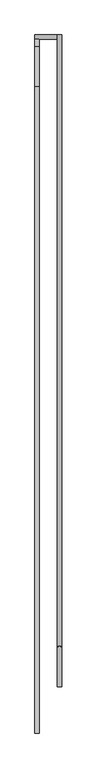
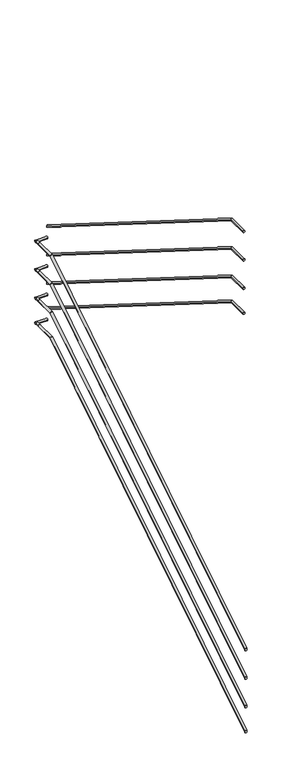
"""IFC4 building model written with IfcOpenShell, lengths in millimetres: railing geometry."""

from ifc_helpers import new_model, si_unit, frame, origin, place, context, project, spatial, circle_curve, ellipse_curve, source, transform, mapped, element, save
from ifc_brep_helpers import plane_surface, cylinder_surface, advanced_brep


def railing_b70a03e3(model_context):
    return source(origin(), model_context, "Body", "AdvancedBrep", [
        advanced_brep(
        [(52769.6, 10964.5208589, 1508.0091814), (52799.6, 10964.5208589, 1508.0091814), (52769.6, 15448.8385799, 4322.8406512), (52799.6, 15448.8385799, 4322.8406512), (52769.6, 15724.5208589, 4322.8406512), (52799.6, 15724.5208589, 4322.8406512)],
        [
            (0, 1, ellipse_curve(frame((52784.6, 10964.5208589, 1508.0091814), z_axis=(0.0, -1.0, 0.0), x_axis=(0.0, 0.0, -1.0)), 17.7102578, 15.0)),
            (1, 0, ellipse_curve(frame((52784.6, 10964.5208589, 1508.0091814), z_axis=(0.0, -1.0, 0.0), x_axis=(0.0, 0.0, -1.0)), 17.7102578, 15.0)),
            (0, 2),
            (2, 3, ellipse_curve(frame((52784.6, 15448.8385799, 4322.8406512), z_axis=(0.0, -0.9609804318330746, -0.27661635821823227), x_axis=(0.0, 0.27661635821823216, -0.9609804318330747)), 15.6090587, 15.0)),
            (3, 1),
            (3, 2, ellipse_curve(frame((52784.6, 15448.8385799, 4322.8406512), z_axis=(0.0, -0.9609804318330746, -0.27661635821823227), x_axis=(0.0, 0.27661635821823216, -0.9609804318330747)), 15.6090587, 15.0)),
            (4, 5, circle_curve(frame((52784.6, 15724.5208589, 4322.8406512), z_axis=(0.0, 1.0, 0.0), x_axis=(1.0, 0.0, 0.0)), 15.0)),
            (5, 4, circle_curve(frame((52784.6, 15724.5208589, 4322.8406512), z_axis=(0.0, 1.0, 0.0), x_axis=(1.0, 0.0, 0.0)), 15.0)),
            (2, 4),
            (5, 3),
        ],
        [
            plane_surface(frame((52784.6, 10964.5208589, 1525.7194391), z_axis=(0.0, -1.0, 0.0), x_axis=(0.0, 0.0, 1.0))),
            cylinder_surface(frame((52784.6, 10972.4955461, 1513.0149374), z_axis=(0.0, -0.8469667807321652, -0.5316458147452987), x_axis=(1.0, 0.0, 0.0)), 15.0),
            plane_surface(frame((52784.6, 15724.5208589, 4337.8406512), z_axis=(0.0, 1.0, 0.0), x_axis=(0.0, 0.0, 1.0))),
            cylinder_surface(frame((52784.6, 15444.5208589, 4322.8406512), z_axis=(0.0, -1.0, 0.0), x_axis=(1.0, 0.0, 0.0)), 15.0),
        ],
        [
            (0, [[1, 2]]),
            (1, [[-1, 3, 4, 5]]),
            (1, [[-2, -5, 6, -3]]),
            (2, [[7, 8]]),
            (3, [[-4, 9, -8, 10]]),
            (3, [[-6, -10, -7, -9]]),
        ],
    ),
        advanced_brep(
        [(52769.6, 15724.5208589, 4322.8406512), (52799.6, 15724.5208589, 4322.8406512), (52769.6, 15774.9208589, 4322.8406512), (52799.6, 15774.9208589, 4322.8406512)],
        [
            (0, 1, circle_curve(frame((52784.6, 15724.5208589, 4322.8406512), z_axis=(0.0, -1.0, 0.0), x_axis=(1.0, 0.0, 0.0)), 15.0)),
            (1, 0, circle_curve(frame((52784.6, 15724.5208589, 4322.8406512), z_axis=(0.0, -1.0, 0.0), x_axis=(1.0, 0.0, 0.0)), 15.0)),
            (2, 3, circle_curve(frame((52784.6, 15774.9208589, 4322.8406512), z_axis=(0.0, 1.0, 0.0), x_axis=(1.0, 0.0, 0.0)), 15.0)),
            (3, 2, circle_curve(frame((52784.6, 15774.9208589, 4322.8406512), z_axis=(0.0, 1.0, 0.0), x_axis=(1.0, 0.0, 0.0)), 15.0)),
            (0, 2),
            (3, 1),
        ],
        [
            plane_surface(frame((52784.6, 15724.5208589, 4337.8406512), z_axis=(0.0, -1.0, 0.0), x_axis=(0.0, 0.0, 1.0))),
            plane_surface(frame((52784.6, 15774.9208589, 4337.8406512), z_axis=(0.0, 1.0, 0.0), x_axis=(0.0, 0.0, 1.0))),
            cylinder_surface(frame((52784.6, 15724.5208589, 4322.8406512), z_axis=(0.0, -1.0, 0.0), x_axis=(1.0, 0.0, 0.0)), 15.0),
        ],
        [
            (0, [[1, 2]]),
            (1, [[3, 4]]),
            (2, [[-1, 5, -4, 6]]),
            (2, [[-2, -6, -3, -5]]),
        ],
    ),
        advanced_brep(
        [(52769.6, 15804.9208589, 4322.8406512), (52769.6, 15774.9208589, 4322.8406512), (52925.4, 15804.9208589, 4322.8406512), (52925.4, 15774.9208589, 4322.8406512)],
        [
            (0, 1, circle_curve(frame((52769.6, 15789.9208589, 4322.8406512), z_axis=(-1.0, 0.0, 0.0), x_axis=(0.0, -1.0, 0.0)), 15.0)),
            (1, 0, circle_curve(frame((52769.6, 15789.9208589, 4322.8406512), z_axis=(-1.0, 0.0, 0.0), x_axis=(0.0, -1.0, 0.0)), 15.0)),
            (2, 3, circle_curve(frame((52925.4, 15789.9208589, 4322.8406512), z_axis=(1.0, 0.0, 0.0), x_axis=(0.0, -1.0, 0.0)), 15.0)),
            (3, 2, circle_curve(frame((52925.4, 15789.9208589, 4322.8406512), z_axis=(1.0, 0.0, 0.0), x_axis=(0.0, -1.0, 0.0)), 15.0)),
            (0, 2),
            (3, 1),
        ],
        [
            plane_surface(frame((52769.6, 15789.9208589, 4337.8406512), z_axis=(-1.0, 0.0, 0.0), x_axis=(0.0, 1.0, 0.0))),
            plane_surface(frame((52925.4, 15789.9208589, 4337.8406512), z_axis=(1.0, 0.0, 0.0), x_axis=(0.0, 1.0, 0.0))),
            cylinder_surface(frame((52769.6, 15789.9208589, 4322.8406512), z_axis=(-1.0, 0.0, 0.0), x_axis=(0.0, -1.0, 0.0)), 15.0),
        ],
        [
            (0, [[1, 2]]),
            (1, [[3, 4]]),
            (2, [[-1, 5, -4, 6]]),
            (2, [[-2, -6, -3, -5]]),
        ],
    ),
        advanced_brep(
        [(52955.4, 15804.9208589, 4470.5286619), (52925.4, 15804.9208589, 4470.5286619), (52955.4, 11560.2031379, 7134.9618634), (52925.4, 11560.2031379, 7134.9618634), (52955.4, 11284.5208589, 7134.9618634), (52925.4, 11284.5208589, 7134.9618634)],
        [
            (0, 1, ellipse_curve(frame((52940.4, 15804.9208589, 4470.5286619), z_axis=(0.0, 1.0, 0.0), x_axis=(0.0, 0.0, -1.0)), 17.7102578, 15.0)),
            (1, 0, ellipse_curve(frame((52940.4, 15804.9208589, 4470.5286619), z_axis=(0.0, 1.0, 0.0), x_axis=(0.0, 0.0, -1.0)), 17.7102578, 15.0)),
            (0, 2),
            (2, 3, ellipse_curve(frame((52940.4, 11560.2031379, 7134.9618634), z_axis=(0.0, 0.9609804318330746, -0.2766163582182322), x_axis=(0.0, -0.2766163582182318, -0.9609804318330748)), 15.6090587, 15.0)),
            (3, 1),
            (3, 2, ellipse_curve(frame((52940.4, 11560.2031379, 7134.9618634), z_axis=(0.0, 0.9609804318330746, -0.2766163582182322), x_axis=(0.0, -0.2766163582182318, -0.9609804318330748)), 15.6090587, 15.0)),
            (4, 5, circle_curve(frame((52940.4, 11284.5208589, 7134.9618634), z_axis=(0.0, -1.0, 0.0), x_axis=(-1.0, 0.0, 0.0)), 15.0)),
            (5, 4, circle_curve(frame((52940.4, 11284.5208589, 7134.9618634), z_axis=(0.0, -1.0, 0.0), x_axis=(-1.0, 0.0, 0.0)), 15.0)),
            (2, 4),
            (5, 3),
        ],
        [
            plane_surface(frame((52940.4, 15804.9208589, 4488.2389196), z_axis=(0.0, 1.0, 0.0), x_axis=(0.0, 0.0, -1.0))),
            cylinder_surface(frame((52940.4, 15796.9461717, 4475.5344179), z_axis=(0.0, 0.8469667807321652, -0.5316458147452986), x_axis=(-1.0, 0.0, 0.0)), 15.0),
            plane_surface(frame((52940.4, 11284.5208589, 7149.9618634), z_axis=(0.0, -1.0, 0.0), x_axis=(0.0, 0.0, -1.0))),
            cylinder_surface(frame((52940.4, 11564.5208589, 7134.9618634), z_axis=(0.0, 1.0, 0.0), x_axis=(-1.0, 0.0, 0.0)), 15.0),
        ],
        [
            (0, [[1, 2]]),
            (1, [[-1, 3, 4, 5]]),
            (1, [[-2, -5, 6, -3]]),
            (2, [[7, 8]]),
            (3, [[-4, 9, -8, 10]]),
            (3, [[-6, -10, -7, -9]]),
        ],
    ),
        advanced_brep(
        [(52769.6, 10964.5208589, 708.0091814), (52799.6, 10964.5208589, 708.0091814), (52769.6, 15448.8385799, 3522.8406512), (52799.6, 15448.8385799, 3522.8406512), (52769.6, 15724.5208589, 3522.8406512), (52799.6, 15724.5208589, 3522.8406512)],
        [
            (0, 1, ellipse_curve(frame((52784.6, 10964.5208589, 708.0091814), z_axis=(0.0, -1.0, 0.0), x_axis=(0.0, 0.0, -1.0)), 17.7102578, 15.0)),
            (1, 0, ellipse_curve(frame((52784.6, 10964.5208589, 708.0091814), z_axis=(0.0, -1.0, 0.0), x_axis=(0.0, 0.0, -1.0)), 17.7102578, 15.0)),
            (0, 2),
            (2, 3, ellipse_curve(frame((52784.6, 15448.8385799, 3522.8406512), z_axis=(0.0, -0.9609804318330746, -0.27661635821823227), x_axis=(0.0, 0.27661635821823216, -0.9609804318330747)), 15.6090587, 15.0)),
            (3, 1),
            (3, 2, ellipse_curve(frame((52784.6, 15448.8385799, 3522.8406512), z_axis=(0.0, -0.9609804318330746, -0.27661635821823227), x_axis=(0.0, 0.27661635821823216, -0.9609804318330747)), 15.6090587, 15.0)),
            (4, 5, circle_curve(frame((52784.6, 15724.5208589, 3522.8406512), z_axis=(0.0, 1.0, 0.0), x_axis=(1.0, 0.0, 0.0)), 15.0)),
            (5, 4, circle_curve(frame((52784.6, 15724.5208589, 3522.8406512), z_axis=(0.0, 1.0, 0.0), x_axis=(1.0, 0.0, 0.0)), 15.0)),
            (2, 4),
            (5, 3),
        ],
        [
            plane_surface(frame((52784.6, 10964.5208589, 725.7194391), z_axis=(0.0, -1.0, 0.0), x_axis=(0.0, 0.0, 1.0))),
            cylinder_surface(frame((52784.6, 10972.4955461, 713.0149374), z_axis=(0.0, -0.8469667807321652, -0.5316458147452987), x_axis=(1.0, 0.0, 0.0)), 15.0),
            plane_surface(frame((52784.6, 15724.5208589, 3537.8406512), z_axis=(0.0, 1.0, 0.0), x_axis=(0.0, 0.0, 1.0))),
            cylinder_surface(frame((52784.6, 15444.5208589, 3522.8406512), z_axis=(0.0, -1.0, 0.0), x_axis=(1.0, 0.0, 0.0)), 15.0),
        ],
        [
            (0, [[1, 2]]),
            (1, [[-1, 3, 4, 5]]),
            (1, [[-2, -5, 6, -3]]),
            (2, [[7, 8]]),
            (3, [[-4, 9, -8, 10]]),
            (3, [[-6, -10, -7, -9]]),
        ],
    ),
        advanced_brep(
        [(52769.6, 15724.5208589, 3522.8406512), (52799.6, 15724.5208589, 3522.8406512), (52769.6, 15774.9208589, 3522.8406512), (52799.6, 15774.9208589, 3522.8406512)],
        [
            (0, 1, circle_curve(frame((52784.6, 15724.5208589, 3522.8406512), z_axis=(0.0, -1.0, 0.0), x_axis=(1.0, 0.0, 0.0)), 15.0)),
            (1, 0, circle_curve(frame((52784.6, 15724.5208589, 3522.8406512), z_axis=(0.0, -1.0, 0.0), x_axis=(1.0, 0.0, 0.0)), 15.0)),
            (2, 3, circle_curve(frame((52784.6, 15774.9208589, 3522.8406512), z_axis=(0.0, 1.0, 0.0), x_axis=(1.0, 0.0, 0.0)), 15.0)),
            (3, 2, circle_curve(frame((52784.6, 15774.9208589, 3522.8406512), z_axis=(0.0, 1.0, 0.0), x_axis=(1.0, 0.0, 0.0)), 15.0)),
            (0, 2),
            (3, 1),
        ],
        [
            plane_surface(frame((52784.6, 15724.5208589, 3537.8406512), z_axis=(0.0, -1.0, 0.0), x_axis=(0.0, 0.0, 1.0))),
            plane_surface(frame((52784.6, 15774.9208589, 3537.8406512), z_axis=(0.0, 1.0, 0.0), x_axis=(0.0, 0.0, 1.0))),
            cylinder_surface(frame((52784.6, 15724.5208589, 3522.8406512), z_axis=(0.0, -1.0, 0.0), x_axis=(1.0, 0.0, 0.0)), 15.0),
        ],
        [
            (0, [[1, 2]]),
            (1, [[3, 4]]),
            (2, [[-1, 5, -4, 6]]),
            (2, [[-2, -6, -3, -5]]),
        ],
    ),
        advanced_brep(
        [(52769.6, 15804.9208589, 3522.8406512), (52769.6, 15774.9208589, 3522.8406512), (52925.4, 15804.9208589, 3522.8406512), (52925.4, 15774.9208589, 3522.8406512)],
        [
            (0, 1, circle_curve(frame((52769.6, 15789.9208589, 3522.8406512), z_axis=(-1.0, 0.0, 0.0), x_axis=(0.0, -1.0, 0.0)), 15.0)),
            (1, 0, circle_curve(frame((52769.6, 15789.9208589, 3522.8406512), z_axis=(-1.0, 0.0, 0.0), x_axis=(0.0, -1.0, 0.0)), 15.0)),
            (2, 3, circle_curve(frame((52925.4, 15789.9208589, 3522.8406512), z_axis=(1.0, 0.0, 0.0), x_axis=(0.0, -1.0, 0.0)), 15.0)),
            (3, 2, circle_curve(frame((52925.4, 15789.9208589, 3522.8406512), z_axis=(1.0, 0.0, 0.0), x_axis=(0.0, -1.0, 0.0)), 15.0)),
            (0, 2),
            (3, 1),
        ],
        [
            plane_surface(frame((52769.6, 15789.9208589, 3537.8406512), z_axis=(-1.0, 0.0, 0.0), x_axis=(0.0, 1.0, 0.0))),
            plane_surface(frame((52925.4, 15789.9208589, 3537.8406512), z_axis=(1.0, 0.0, 0.0), x_axis=(0.0, 1.0, 0.0))),
            cylinder_surface(frame((52769.6, 15789.9208589, 3522.8406512), z_axis=(-1.0, 0.0, 0.0), x_axis=(0.0, -1.0, 0.0)), 15.0),
        ],
        [
            (0, [[1, 2]]),
            (1, [[3, 4]]),
            (2, [[-1, 5, -4, 6]]),
            (2, [[-2, -6, -3, -5]]),
        ],
    ),
        advanced_brep(
        [(52955.4, 15804.9208589, 3670.5286619), (52925.4, 15804.9208589, 3670.5286619), (52955.4, 11560.2031379, 6334.9618634), (52925.4, 11560.2031379, 6334.9618634), (52955.4, 11284.5208589, 6334.9618634), (52925.4, 11284.5208589, 6334.9618634)],
        [
            (0, 1, ellipse_curve(frame((52940.4, 15804.9208589, 3670.5286619), z_axis=(0.0, 1.0, 0.0), x_axis=(0.0, 0.0, -1.0)), 17.7102578, 15.0)),
            (1, 0, ellipse_curve(frame((52940.4, 15804.9208589, 3670.5286619), z_axis=(0.0, 1.0, 0.0), x_axis=(0.0, 0.0, -1.0)), 17.7102578, 15.0)),
            (0, 2),
            (2, 3, ellipse_curve(frame((52940.4, 11560.2031379, 6334.9618634), z_axis=(0.0, 0.9609804318330746, -0.2766163582182322), x_axis=(0.0, -0.2766163582182318, -0.9609804318330748)), 15.6090587, 15.0)),
            (3, 1),
            (3, 2, ellipse_curve(frame((52940.4, 11560.2031379, 6334.9618634), z_axis=(0.0, 0.9609804318330746, -0.2766163582182322), x_axis=(0.0, -0.2766163582182318, -0.9609804318330748)), 15.6090587, 15.0)),
            (4, 5, circle_curve(frame((52940.4, 11284.5208589, 6334.9618634), z_axis=(0.0, -1.0, 0.0), x_axis=(-1.0, 0.0, 0.0)), 15.0)),
            (5, 4, circle_curve(frame((52940.4, 11284.5208589, 6334.9618634), z_axis=(0.0, -1.0, 0.0), x_axis=(-1.0, 0.0, 0.0)), 15.0)),
            (2, 4),
            (5, 3),
        ],
        [
            plane_surface(frame((52940.4, 15804.9208589, 3688.2389196), z_axis=(0.0, 1.0, 0.0), x_axis=(0.0, 0.0, -1.0))),
            cylinder_surface(frame((52940.4, 15796.9461717, 3675.5344179), z_axis=(0.0, 0.8469667807321652, -0.5316458147452986), x_axis=(-1.0, 0.0, 0.0)), 15.0),
            plane_surface(frame((52940.4, 11284.5208589, 6349.9618634), z_axis=(0.0, -1.0, 0.0), x_axis=(0.0, 0.0, -1.0))),
            cylinder_surface(frame((52940.4, 11564.5208589, 6334.9618634), z_axis=(0.0, 1.0, 0.0), x_axis=(-1.0, 0.0, 0.0)), 15.0),
        ],
        [
            (0, [[1, 2]]),
            (1, [[-1, 3, 4, 5]]),
            (1, [[-2, -5, 6, -3]]),
            (2, [[7, 8]]),
            (3, [[-4, 9, -8, 10]]),
            (3, [[-6, -10, -7, -9]]),
        ],
    ),
        advanced_brep(
        [(52769.6, 10964.5208589, 1108.0091814), (52799.6, 10964.5208589, 1108.0091814), (52769.6, 15448.8385799, 3922.8406512), (52799.6, 15448.8385799, 3922.8406512), (52769.6, 15724.5208589, 3922.8406512), (52799.6, 15724.5208589, 3922.8406512)],
        [
            (0, 1, ellipse_curve(frame((52784.6, 10964.5208589, 1108.0091814), z_axis=(0.0, -1.0, 0.0), x_axis=(0.0, 0.0, -1.0)), 17.7102578, 15.0)),
            (1, 0, ellipse_curve(frame((52784.6, 10964.5208589, 1108.0091814), z_axis=(0.0, -1.0, 0.0), x_axis=(0.0, 0.0, -1.0)), 17.7102578, 15.0)),
            (0, 2),
            (2, 3, ellipse_curve(frame((52784.6, 15448.8385799, 3922.8406512), z_axis=(0.0, -0.9609804318330746, -0.27661635821823227), x_axis=(0.0, 0.27661635821823216, -0.9609804318330747)), 15.6090587, 15.0)),
            (3, 1),
            (3, 2, ellipse_curve(frame((52784.6, 15448.8385799, 3922.8406512), z_axis=(0.0, -0.9609804318330746, -0.27661635821823227), x_axis=(0.0, 0.27661635821823216, -0.9609804318330747)), 15.6090587, 15.0)),
            (4, 5, circle_curve(frame((52784.6, 15724.5208589, 3922.8406512), z_axis=(0.0, 1.0, 0.0), x_axis=(1.0, 0.0, 0.0)), 15.0)),
            (5, 4, circle_curve(frame((52784.6, 15724.5208589, 3922.8406512), z_axis=(0.0, 1.0, 0.0), x_axis=(1.0, 0.0, 0.0)), 15.0)),
            (2, 4),
            (5, 3),
        ],
        [
            plane_surface(frame((52784.6, 10964.5208589, 1125.7194391), z_axis=(0.0, -1.0, 0.0), x_axis=(0.0, 0.0, 1.0))),
            cylinder_surface(frame((52784.6, 10972.4955461, 1113.0149374), z_axis=(0.0, -0.8469667807321652, -0.5316458147452987), x_axis=(1.0, 0.0, 0.0)), 15.0),
            plane_surface(frame((52784.6, 15724.5208589, 3937.8406512), z_axis=(0.0, 1.0, 0.0), x_axis=(0.0, 0.0, 1.0))),
            cylinder_surface(frame((52784.6, 15444.5208589, 3922.8406512), z_axis=(0.0, -1.0, 0.0), x_axis=(1.0, 0.0, 0.0)), 15.0),
        ],
        [
            (0, [[1, 2]]),
            (1, [[-1, 3, 4, 5]]),
            (1, [[-2, -5, 6, -3]]),
            (2, [[7, 8]]),
            (3, [[-4, 9, -8, 10]]),
            (3, [[-6, -10, -7, -9]]),
        ],
    ),
        advanced_brep(
        [(52769.6, 15724.5208589, 3922.8406512), (52799.6, 15724.5208589, 3922.8406512), (52769.6, 15774.9208589, 3922.8406512), (52799.6, 15774.9208589, 3922.8406512)],
        [
            (0, 1, circle_curve(frame((52784.6, 15724.5208589, 3922.8406512), z_axis=(0.0, -1.0, 0.0), x_axis=(1.0, 0.0, 0.0)), 15.0)),
            (1, 0, circle_curve(frame((52784.6, 15724.5208589, 3922.8406512), z_axis=(0.0, -1.0, 0.0), x_axis=(1.0, 0.0, 0.0)), 15.0)),
            (2, 3, circle_curve(frame((52784.6, 15774.9208589, 3922.8406512), z_axis=(0.0, 1.0, 0.0), x_axis=(1.0, 0.0, 0.0)), 15.0)),
            (3, 2, circle_curve(frame((52784.6, 15774.9208589, 3922.8406512), z_axis=(0.0, 1.0, 0.0), x_axis=(1.0, 0.0, 0.0)), 15.0)),
            (0, 2),
            (3, 1),
        ],
        [
            plane_surface(frame((52784.6, 15724.5208589, 3937.8406512), z_axis=(0.0, -1.0, 0.0), x_axis=(0.0, 0.0, 1.0))),
            plane_surface(frame((52784.6, 15774.9208589, 3937.8406512), z_axis=(0.0, 1.0, 0.0), x_axis=(0.0, 0.0, 1.0))),
            cylinder_surface(frame((52784.6, 15724.5208589, 3922.8406512), z_axis=(0.0, -1.0, 0.0), x_axis=(1.0, 0.0, 0.0)), 15.0),
        ],
        [
            (0, [[1, 2]]),
            (1, [[3, 4]]),
            (2, [[-1, 5, -4, 6]]),
            (2, [[-2, -6, -3, -5]]),
        ],
    ),
        advanced_brep(
        [(52769.6, 15804.9208589, 3922.8406512), (52769.6, 15774.9208589, 3922.8406512), (52925.4, 15804.9208589, 3922.8406512), (52925.4, 15774.9208589, 3922.8406512)],
        [
            (0, 1, circle_curve(frame((52769.6, 15789.9208589, 3922.8406512), z_axis=(-1.0, 0.0, 0.0), x_axis=(0.0, -1.0, 0.0)), 15.0)),
            (1, 0, circle_curve(frame((52769.6, 15789.9208589, 3922.8406512), z_axis=(-1.0, 0.0, 0.0), x_axis=(0.0, -1.0, 0.0)), 15.0)),
            (2, 3, circle_curve(frame((52925.4, 15789.9208589, 3922.8406512), z_axis=(1.0, 0.0, 0.0), x_axis=(0.0, -1.0, 0.0)), 15.0)),
            (3, 2, circle_curve(frame((52925.4, 15789.9208589, 3922.8406512), z_axis=(1.0, 0.0, 0.0), x_axis=(0.0, -1.0, 0.0)), 15.0)),
            (0, 2),
            (3, 1),
        ],
        [
            plane_surface(frame((52769.6, 15789.9208589, 3937.8406512), z_axis=(-1.0, 0.0, 0.0), x_axis=(0.0, 1.0, 0.0))),
            plane_surface(frame((52925.4, 15789.9208589, 3937.8406512), z_axis=(1.0, 0.0, 0.0), x_axis=(0.0, 1.0, 0.0))),
            cylinder_surface(frame((52769.6, 15789.9208589, 3922.8406512), z_axis=(-1.0, 0.0, 0.0), x_axis=(0.0, -1.0, 0.0)), 15.0),
        ],
        [
            (0, [[1, 2]]),
            (1, [[3, 4]]),
            (2, [[-1, 5, -4, 6]]),
            (2, [[-2, -6, -3, -5]]),
        ],
    ),
        advanced_brep(
        [(52955.4, 15804.9208589, 4070.5286619), (52925.4, 15804.9208589, 4070.5286619), (52955.4, 11560.2031379, 6734.9618634), (52925.4, 11560.2031379, 6734.9618634), (52955.4, 11284.5208589, 6734.9618634), (52925.4, 11284.5208589, 6734.9618634)],
        [
            (0, 1, ellipse_curve(frame((52940.4, 15804.9208589, 4070.5286619), z_axis=(0.0, 1.0, 0.0), x_axis=(0.0, 0.0, -1.0)), 17.7102578, 15.0)),
            (1, 0, ellipse_curve(frame((52940.4, 15804.9208589, 4070.5286619), z_axis=(0.0, 1.0, 0.0), x_axis=(0.0, 0.0, -1.0)), 17.7102578, 15.0)),
            (0, 2),
            (2, 3, ellipse_curve(frame((52940.4, 11560.2031379, 6734.9618634), z_axis=(0.0, 0.9609804318330746, -0.2766163582182322), x_axis=(0.0, -0.2766163582182318, -0.9609804318330748)), 15.6090587, 15.0)),
            (3, 1),
            (3, 2, ellipse_curve(frame((52940.4, 11560.2031379, 6734.9618634), z_axis=(0.0, 0.9609804318330746, -0.2766163582182322), x_axis=(0.0, -0.2766163582182318, -0.9609804318330748)), 15.6090587, 15.0)),
            (4, 5, circle_curve(frame((52940.4, 11284.5208589, 6734.9618634), z_axis=(0.0, -1.0, 0.0), x_axis=(-1.0, 0.0, 0.0)), 15.0)),
            (5, 4, circle_curve(frame((52940.4, 11284.5208589, 6734.9618634), z_axis=(0.0, -1.0, 0.0), x_axis=(-1.0, 0.0, 0.0)), 15.0)),
            (2, 4),
            (5, 3),
        ],
        [
            plane_surface(frame((52940.4, 15804.9208589, 4088.2389196), z_axis=(0.0, 1.0, 0.0), x_axis=(0.0, 0.0, -1.0))),
            cylinder_surface(frame((52940.4, 15796.9461717, 4075.5344179), z_axis=(0.0, 0.8469667807321652, -0.5316458147452986), x_axis=(-1.0, 0.0, 0.0)), 15.0),
            plane_surface(frame((52940.4, 11284.5208589, 6749.9618634), z_axis=(0.0, -1.0, 0.0), x_axis=(0.0, 0.0, -1.0))),
            cylinder_surface(frame((52940.4, 11564.5208589, 6734.9618634), z_axis=(0.0, 1.0, 0.0), x_axis=(-1.0, 0.0, 0.0)), 15.0),
        ],
        [
            (0, [[1, 2]]),
            (1, [[-1, 3, 4, 5]]),
            (1, [[-2, -5, 6, -3]]),
            (2, [[7, 8]]),
            (3, [[-4, 9, -8, 10]]),
            (3, [[-6, -10, -7, -9]]),
        ],
    ),
        advanced_brep(
        [(52769.6, 10964.5208589, 358.0091814), (52799.6, 10964.5208589, 358.0091814), (52769.6, 15448.8385799, 3172.8406512), (52799.6, 15448.8385799, 3172.8406512), (52769.6, 15724.5208589, 3172.8406512), (52799.6, 15724.5208589, 3172.8406512)],
        [
            (0, 1, ellipse_curve(frame((52784.6, 10964.5208589, 358.0091814), z_axis=(0.0, -1.0, 0.0), x_axis=(0.0, 0.0, -1.0)), 17.7102578, 15.0)),
            (1, 0, ellipse_curve(frame((52784.6, 10964.5208589, 358.0091814), z_axis=(0.0, -1.0, 0.0), x_axis=(0.0, 0.0, -1.0)), 17.7102578, 15.0)),
            (0, 2),
            (2, 3, ellipse_curve(frame((52784.6, 15448.8385799, 3172.8406512), z_axis=(0.0, -0.9609804318330746, -0.27661635821823227), x_axis=(0.0, 0.27661635821823216, -0.9609804318330747)), 15.6090587, 15.0)),
            (3, 1),
            (3, 2, ellipse_curve(frame((52784.6, 15448.8385799, 3172.8406512), z_axis=(0.0, -0.9609804318330746, -0.27661635821823227), x_axis=(0.0, 0.27661635821823216, -0.9609804318330747)), 15.6090587, 15.0)),
            (4, 5, circle_curve(frame((52784.6, 15724.5208589, 3172.8406512), z_axis=(0.0, 1.0, 0.0), x_axis=(1.0, 0.0, 0.0)), 15.0)),
            (5, 4, circle_curve(frame((52784.6, 15724.5208589, 3172.8406512), z_axis=(0.0, 1.0, 0.0), x_axis=(1.0, 0.0, 0.0)), 15.0)),
            (2, 4),
            (5, 3),
        ],
        [
            plane_surface(frame((52784.6, 10964.5208589, 375.7194391), z_axis=(0.0, -1.0, 0.0), x_axis=(0.0, 0.0, 1.0))),
            cylinder_surface(frame((52784.6, 10972.4955461, 363.0149374), z_axis=(0.0, -0.8469667807321652, -0.5316458147452987), x_axis=(1.0, 0.0, 0.0)), 15.0),
            plane_surface(frame((52784.6, 15724.5208589, 3187.8406512), z_axis=(0.0, 1.0, 0.0), x_axis=(0.0, 0.0, 1.0))),
            cylinder_surface(frame((52784.6, 15444.5208589, 3172.8406512), z_axis=(0.0, -1.0, 0.0), x_axis=(1.0, 0.0, 0.0)), 15.0),
        ],
        [
            (0, [[1, 2]]),
            (1, [[-1, 3, 4, 5]]),
            (1, [[-2, -5, 6, -3]]),
            (2, [[7, 8]]),
            (3, [[-4, 9, -8, 10]]),
            (3, [[-6, -10, -7, -9]]),
        ],
    ),
        advanced_brep(
        [(52769.6, 15724.5208589, 3172.8406512), (52799.6, 15724.5208589, 3172.8406512), (52769.6, 15774.9208589, 3172.8406512), (52799.6, 15774.9208589, 3172.8406512)],
        [
            (0, 1, circle_curve(frame((52784.6, 15724.5208589, 3172.8406512), z_axis=(0.0, -1.0, 0.0), x_axis=(1.0, 0.0, 0.0)), 15.0)),
            (1, 0, circle_curve(frame((52784.6, 15724.5208589, 3172.8406512), z_axis=(0.0, -1.0, 0.0), x_axis=(1.0, 0.0, 0.0)), 15.0)),
            (2, 3, circle_curve(frame((52784.6, 15774.9208589, 3172.8406512), z_axis=(0.0, 1.0, 0.0), x_axis=(1.0, 0.0, 0.0)), 15.0)),
            (3, 2, circle_curve(frame((52784.6, 15774.9208589, 3172.8406512), z_axis=(0.0, 1.0, 0.0), x_axis=(1.0, 0.0, 0.0)), 15.0)),
            (0, 2),
            (3, 1),
        ],
        [
            plane_surface(frame((52784.6, 15724.5208589, 3187.8406512), z_axis=(0.0, -1.0, 0.0), x_axis=(0.0, 0.0, 1.0))),
            plane_surface(frame((52784.6, 15774.9208589, 3187.8406512), z_axis=(0.0, 1.0, 0.0), x_axis=(0.0, 0.0, 1.0))),
            cylinder_surface(frame((52784.6, 15724.5208589, 3172.8406512), z_axis=(0.0, -1.0, 0.0), x_axis=(1.0, 0.0, 0.0)), 15.0),
        ],
        [
            (0, [[1, 2]]),
            (1, [[3, 4]]),
            (2, [[-1, 5, -4, 6]]),
            (2, [[-2, -6, -3, -5]]),
        ],
    ),
        advanced_brep(
        [(52769.6, 15804.9208589, 3172.8406512), (52769.6, 15774.9208589, 3172.8406512), (52925.4, 15804.9208589, 3172.8406512), (52925.4, 15774.9208589, 3172.8406512)],
        [
            (0, 1, circle_curve(frame((52769.6, 15789.9208589, 3172.8406512), z_axis=(-1.0, 0.0, 0.0), x_axis=(0.0, -1.0, 0.0)), 15.0)),
            (1, 0, circle_curve(frame((52769.6, 15789.9208589, 3172.8406512), z_axis=(-1.0, 0.0, 0.0), x_axis=(0.0, -1.0, 0.0)), 15.0)),
            (2, 3, circle_curve(frame((52925.4, 15789.9208589, 3172.8406512), z_axis=(1.0, 0.0, 0.0), x_axis=(0.0, -1.0, 0.0)), 15.0)),
            (3, 2, circle_curve(frame((52925.4, 15789.9208589, 3172.8406512), z_axis=(1.0, 0.0, 0.0), x_axis=(0.0, -1.0, 0.0)), 15.0)),
            (0, 2),
            (3, 1),
        ],
        [
            plane_surface(frame((52769.6, 15789.9208589, 3187.8406512), z_axis=(-1.0, 0.0, 0.0), x_axis=(0.0, 1.0, 0.0))),
            plane_surface(frame((52925.4, 15789.9208589, 3187.8406512), z_axis=(1.0, 0.0, 0.0), x_axis=(0.0, 1.0, 0.0))),
            cylinder_surface(frame((52769.6, 15789.9208589, 3172.8406512), z_axis=(-1.0, 0.0, 0.0), x_axis=(0.0, -1.0, 0.0)), 15.0),
        ],
        [
            (0, [[1, 2]]),
            (1, [[3, 4]]),
            (2, [[-1, 5, -4, 6]]),
            (2, [[-2, -6, -3, -5]]),
        ],
    ),
        advanced_brep(
        [(52955.4, 15804.9208589, 3320.5286619), (52925.4, 15804.9208589, 3320.5286619), (52955.4, 11560.2031379, 5984.9618634), (52925.4, 11560.2031379, 5984.9618634), (52955.4, 11284.5208589, 5984.9618634), (52925.4, 11284.5208589, 5984.9618634)],
        [
            (0, 1, ellipse_curve(frame((52940.4, 15804.9208589, 3320.5286619), z_axis=(0.0, 1.0, 0.0), x_axis=(0.0, 0.0, -1.0)), 17.7102578, 15.0)),
            (1, 0, ellipse_curve(frame((52940.4, 15804.9208589, 3320.5286619), z_axis=(0.0, 1.0, 0.0), x_axis=(0.0, 0.0, -1.0)), 17.7102578, 15.0)),
            (0, 2),
            (2, 3, ellipse_curve(frame((52940.4, 11560.2031379, 5984.9618634), z_axis=(0.0, 0.9609804318330746, -0.2766163582182322), x_axis=(0.0, -0.2766163582182318, -0.9609804318330748)), 15.6090587, 15.0)),
            (3, 1),
            (3, 2, ellipse_curve(frame((52940.4, 11560.2031379, 5984.9618634), z_axis=(0.0, 0.9609804318330746, -0.2766163582182322), x_axis=(0.0, -0.2766163582182318, -0.9609804318330748)), 15.6090587, 15.0)),
            (4, 5, circle_curve(frame((52940.4, 11284.5208589, 5984.9618634), z_axis=(0.0, -1.0, 0.0), x_axis=(-1.0, 0.0, 0.0)), 15.0)),
            (5, 4, circle_curve(frame((52940.4, 11284.5208589, 5984.9618634), z_axis=(0.0, -1.0, 0.0), x_axis=(-1.0, 0.0, 0.0)), 15.0)),
            (2, 4),
            (5, 3),
        ],
        [
            plane_surface(frame((52940.4, 15804.9208589, 3338.2389196), z_axis=(0.0, 1.0, 0.0), x_axis=(0.0, 0.0, -1.0))),
            cylinder_surface(frame((52940.4, 15796.9461717, 3325.5344179), z_axis=(0.0, 0.8469667807321652, -0.5316458147452986), x_axis=(-1.0, 0.0, 0.0)), 15.0),
            plane_surface(frame((52940.4, 11284.5208589, 5999.9618634), z_axis=(0.0, -1.0, 0.0), x_axis=(0.0, 0.0, -1.0))),
            cylinder_surface(frame((52940.4, 11564.5208589, 5984.9618634), z_axis=(0.0, 1.0, 0.0), x_axis=(-1.0, 0.0, 0.0)), 15.0),
        ],
        [
            (0, [[1, 2]]),
            (1, [[-1, 3, 4, 5]]),
            (1, [[-2, -5, 6, -3]]),
            (2, [[7, 8]]),
            (3, [[-4, 9, -8, 10]]),
            (3, [[-6, -10, -7, -9]]),
        ],
    ),
    ])


if __name__ == "__main__":
    model = new_model("IFC4")
    model_context = context("Model", 3, world=origin())
    ifc_project = project(units=[si_unit("LENGTHUNIT", "METRE", prefix="MILLI")], contexts=[model_context])
    site = spatial("IfcSite", under=ifc_project)
    building = spatial("IfcBuilding", under=site)
    placement = place(None, origin())
    railing_shape = railing_b70a03e3(model_context)
    element("IfcRailing", 1, at=placement, inside=building, context=model_context, shape_type="MappedRepresentation", body=[
        mapped(railing_shape, transform((0.0, 0.0, 0.0), x_axis=(1.0, 0.0, 0.0), y_axis=(0.0, 1.0, 0.0), z_axis=(0.0, 0.0, 1.0))),
    ])
    save(model, "model.ifc")
